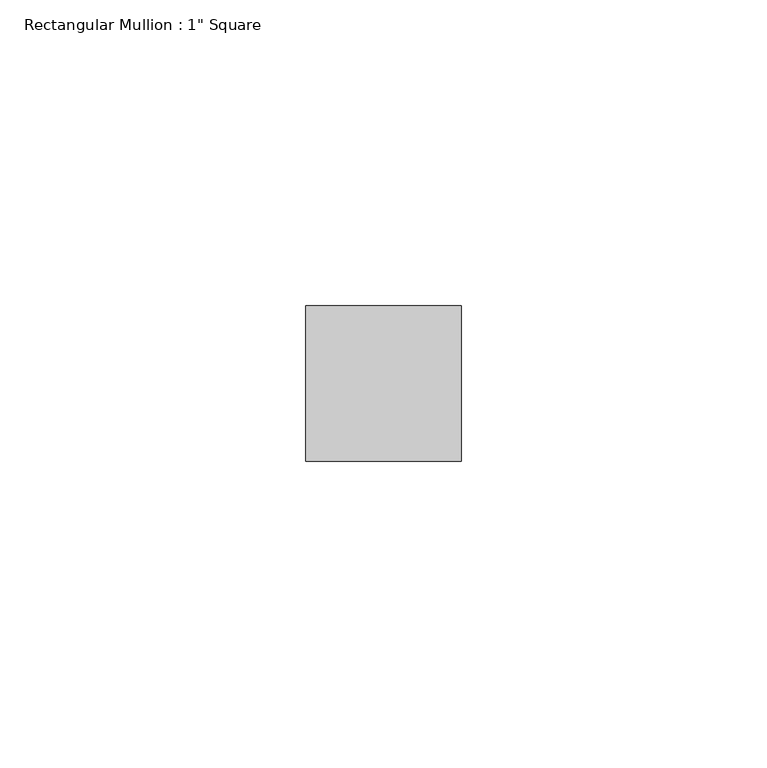
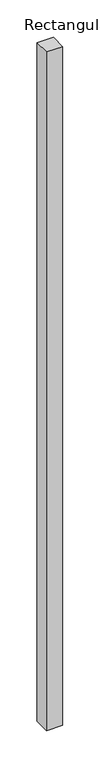
"""IFC4 building model written with IfcOpenShell, lengths in millimetres: member geometry."""

from ifc_helpers import new_model, si_unit, frame, origin, place, context, project, spatial, polyline, outline, extrude, source, transform, mapped, element, save


def member_8f4d6403(model_context):
    return source(origin(), model_context, "Body", "SweptSolid", [
        extrude(outline(polyline([(12.7, 12.7), (12.7, -12.7), (-12.7, -12.7), (-12.7, 12.7), (12.7, 12.7)])), frame((0.0, 0.0, -1115.149828), z_axis=(0.0, 0.0, 1.0), x_axis=(1.0, 0.0, 0.0)), (0.0, 0.0, 1.0), 1115.149828),
    ])


if __name__ == "__main__":
    model = new_model("IFC4")
    model_context = context("Model", 3, world=origin())
    ifc_project = project(units=[si_unit("LENGTHUNIT", "METRE", prefix="MILLI")], contexts=[model_context])
    site = spatial("IfcSite", under=ifc_project)
    building = spatial("IfcBuilding", under=site)
    placement = place(None, origin())
    member_shape = member_8f4d6403(model_context)
    element("IfcMember", 1, ObjectType="Rectangular Mullion : 1\" Square", at=placement, inside=building, context=model_context, shape_type="MappedRepresentation", body=[
        mapped(member_shape, transform((0.0, 0.0, 0.0), x_axis=(1.0, 0.0, 0.0), y_axis=(0.0, 1.0, 0.0), z_axis=(0.0, 0.0, 1.0))),
    ])
    save(model, "model.ifc")

# Revit data of these elements
# Type "Rectangular Mullion : 1\" Square"
#   built-in parameter 1007304 = 0.0833333 (stored number, unit not read)
#   built-in parameter 1007301 = 0.0416667 (stored number, unit not read)
#   built-in parameter 1007300 = 0.0416667 (stored number, unit not read)
# Element 1 (IfcMember, "Rectangular Mullion : 1\" Square")
#   Materials on its faces: "Metal - Aluminum"
# Materials
#   "Metal - Aluminum": class "Metal", colour RGB 247 247 247, transparency 0
